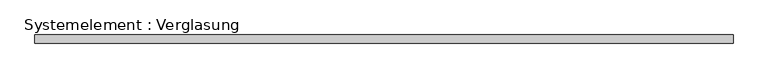
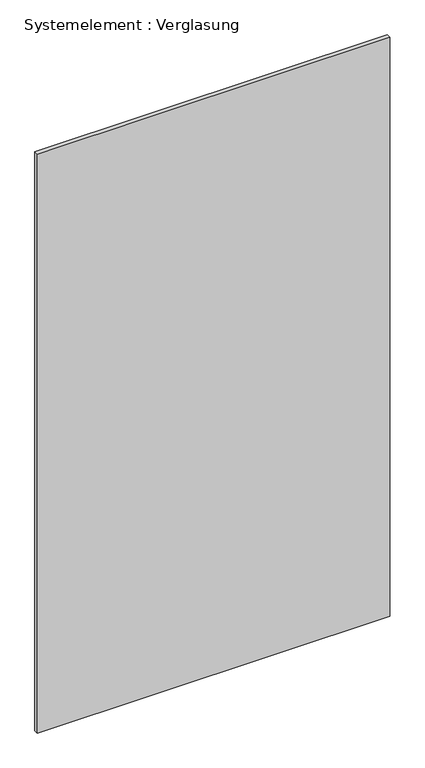
"""IFC4 building model written with IfcOpenShell, lengths in millimetres: plate geometry, Systemelement : Verglasung."""

from ifc_helpers import new_model, si_unit, origin, origin_with_axes, place, context, project, spatial, polyline, outline, extrude, source, transform, mapped, element, save


def systemelement_verglasung_75c3c3d5(model_context):
    return source(origin(), model_context, "Body", "SweptSolid", [
        extrude(outline(polyline([(1220.0, -15.0), (-1220.0, -15.0), (-1220.0, 15.0), (1220.0, 15.0), (1220.0, -15.0)])), origin_with_axes(), (0.0, 0.0, 1.0), 4236.6788019),
    ])


if __name__ == "__main__":
    model = new_model("IFC4")
    model_context = context("Model", 3, world=origin())
    ifc_project = project(units=[si_unit("LENGTHUNIT", "METRE", prefix="MILLI")], contexts=[model_context])
    site = spatial("IfcSite", under=ifc_project)
    building = spatial("IfcBuilding", under=site)
    placement = place(None, origin())
    systemelement_verglasung_shape = systemelement_verglasung_75c3c3d5(model_context)
    element("IfcPlate", 1, ObjectType="Systemelement : Verglasung", at=placement, inside=building, context=model_context, shape_type="MappedRepresentation", body=[
        mapped(systemelement_verglasung_shape, transform((0.0, 0.0, 0.0), x_axis=(1.0, 0.0, 0.0), y_axis=(0.0, 1.0, 0.0), z_axis=(0.0, 0.0, 1.0))),
    ])
    save(model, "model.ifc")

# Revit data of these elements
# Type "Systemelement : Verglasung"
#   Construction Type Id = "GSP4R"
#   Analytic Construction = "1/8 Zoll Pilkington-Verglasung einfach"
#   Visual Light Transmittance = 0.9
#   Solar Heat Gain Coefficient = 0.86
#   Heat Transfer Coefficient (U) = 6.7069 W/(m²·K)
# Element 1 (IfcPlate, "Systemelement : Verglasung")
#   Materials on its faces: "Glas"
# Materials
#   "Glas": class "Glas", colour RGB 0 0 255, transparency 0.75, Comments = "Render-Darstellung nicht aktualisiert ", Cost = 0
